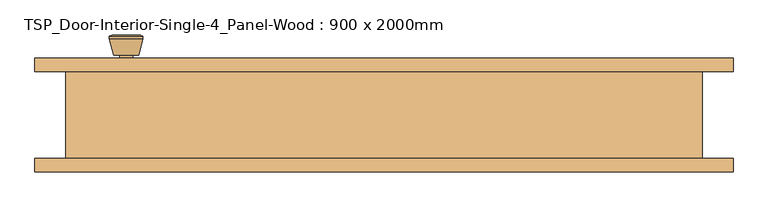
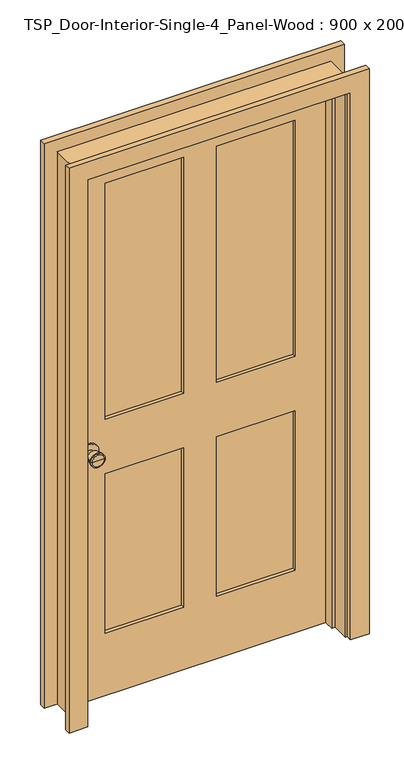
"""IFC4 building model written with IfcOpenShell, lengths in millimetres: door geometry, TSP_Door-Interior-Single-4_Panel-Wood : 900 x 2000mm."""

from ifc_helpers import new_model, si_unit, point, frame, frame_2d, origin, place, context, project, spatial, polyline, circle_curve, trimmed, segment, composite_curve, outline, extrude, faceted_brep, source, transform, mapped, element, save
from ifc_brep_helpers import plane_surface, cylinder_surface, revolved_surface, advanced_brep


def tsp_door_interior_single_4_panel_wood_900_x_2000mm_5c8e3635(model_context):
    return source(origin(), model_context, "Body", "SolidModel", [
        advanced_brep(
        [(-385.0, 20.825, 914.4), (-375.0, 20.825, 914.4), (-395.0, 20.825, 914.4), (-364.5241324, -28.175, 914.4), (-385.0, -28.175, 914.4), (-405.4758676, -28.175, 914.4), (-360.0, -26.3471319, 914.4), (-410.0, -26.3471319, 914.4), (-360.0, -22.8834537, 914.4), (-410.0, -22.8834537, 914.4), (-366.363764, 1.825, 914.4), (-403.636236, 1.825, 914.4), (-375.0, 1.825, 914.4), (-395.0, 1.825, 914.4)],
        [
            (0, 1),
            (1, 2, circle_curve(frame((-385.0, 20.825, 914.4), z_axis=(0.0, 1.0, 0.0), x_axis=(-1.0, 0.0, 0.0)), 10.0)),
            (2, 0),
            (2, 1, circle_curve(frame((-385.0, 20.825, 914.4), z_axis=(0.0, 1.0, 0.0), x_axis=(-1.0, 0.0, 0.0)), 10.0)),
            (3, 4),
            (4, 5),
            (5, 3, circle_curve(frame((-385.0, -28.175, 914.4), z_axis=(0.0, -1.0, 0.0), x_axis=(-1.0, 0.0, 0.0)), 20.4758676)),
            (3, 5, circle_curve(frame((-385.0, -28.175, 914.4), z_axis=(0.0, -1.0, 0.0), x_axis=(-1.0, 0.0, 0.0)), 20.4758676)),
            (6, 3),
            (5, 7),
            (7, 6, circle_curve(frame((-385.0, -26.3471319, 914.4), z_axis=(0.0, -1.0, 0.0), x_axis=(-1.0, 0.0, 0.0)), 25.0)),
            (6, 7, circle_curve(frame((-385.0, -26.3471319, 914.4), z_axis=(0.0, -1.0, 0.0), x_axis=(-1.0, 0.0, 0.0)), 25.0)),
            (8, 6),
            (7, 9),
            (9, 8, circle_curve(frame((-385.0, -22.8834537, 914.4), z_axis=(0.0, -1.0, 0.0), x_axis=(-1.0, 0.0, 0.0)), 25.0)),
            (8, 9, circle_curve(frame((-385.0, -22.8834537, 914.4), z_axis=(0.0, -1.0, 0.0), x_axis=(-1.0, 0.0, 0.0)), 25.0)),
            (10, 8),
            (9, 11),
            (11, 10, circle_curve(frame((-385.0, 1.825, 914.4), z_axis=(0.0, -1.0, 0.0), x_axis=(-1.0, 0.0, 0.0)), 18.636236)),
            (10, 11, circle_curve(frame((-385.0, 1.825, 914.4), z_axis=(0.0, -1.0, 0.0), x_axis=(-1.0, 0.0, 0.0)), 18.636236)),
            (12, 10),
            (11, 13),
            (13, 12, circle_curve(frame((-385.0, 1.825, 914.4), z_axis=(0.0, -1.0, 0.0), x_axis=(-1.0, 0.0, 0.0)), 10.0)),
            (12, 13, circle_curve(frame((-385.0, 1.825, 914.4), z_axis=(0.0, -1.0, 0.0), x_axis=(-1.0, 0.0, 0.0)), 10.0)),
            (1, 12),
            (13, 2),
        ],
        [
            plane_surface(frame((-385.0, 20.825, 914.4), z_axis=(0.0, 1.0, 0.0), x_axis=(-1.0, 0.0, 0.0))),
            plane_surface(frame((-385.0, -28.175, 914.4), z_axis=(0.0, -1.0, 0.0), x_axis=(-1.0, 0.0, 0.0))),
            revolved_surface(polyline([(-405.4758676, -28.175, 914.4), (-410.0, -26.3471319, 914.4)]), (-385.0, 20.825, 914.4), (0.0, 1.0, 0.0)),
            cylinder_surface(frame((-385.0, 20.825, 914.4), z_axis=(0.0, 1.0, 0.0), x_axis=(-1.0, 0.0, 0.0)), 25.0),
            revolved_surface(polyline([(-410.0, -22.8834537, 914.4), (-403.636236, 1.825, 914.4)]), (-385.0, 20.825, 914.4), (0.0, 1.0, 0.0)),
            plane_surface(frame((-385.0, 1.825, 914.4), z_axis=(0.0, 1.0, 0.0), x_axis=(-1.0, 0.0, 0.0))),
            cylinder_surface(frame((-385.0, 20.825, 914.4), z_axis=(0.0, 1.0, 0.0), x_axis=(-1.0, 0.0, 0.0)), 10.0),
        ],
        [
            (0, [[1, 2, 3]]),
            (0, [[-3, 4, -1]]),
            (1, [[5, 6, 7]]),
            (1, [[-6, -5, 8]]),
            (2, [[9, -7, 10, 11]]),
            (2, [[-10, -8, -9, 12]]),
            (3, [[13, -11, 14, 15]]),
            (3, [[-14, -12, -13, 16]]),
            (4, [[17, -15, 18, 19]]),
            (4, [[-18, -16, -17, 20]]),
            (5, [[21, -19, 22, 23]]),
            (5, [[-22, -20, -21, 24]]),
            (6, [[25, -23, 26, -2]]),
            (6, [[-26, -24, -25, -4]]),
        ],
    ),
        extrude(outline(composite_curve([segment(trimmed(circle_curve(frame_2d((914.4, -385.0)), 30.0), [point((914.4, -415.0))], [point((914.4, -355.0))], False, "CARTESIAN"), True, "CONTINUOUS"), segment(trimmed(circle_curve(frame_2d((914.4, -385.0)), 30.0), [point((914.4, -355.0))], [point((914.4, -415.0))], False, "CARTESIAN"), True, "CONTINUOUS")], self_intersect=False)), frame((0.0, 20.825, 0.0), z_axis=(0.0, 1.0, 0.0), x_axis=(0.0, 0.0, 1.0)), (0.0, 0.0, 1.0), 6.0),
        advanced_brep(
        [(-385.0, 67.825, 914.4), (-395.0, 67.825, 914.4), (-375.0, 67.825, 914.4), (-364.5241324, 116.825, 914.4), (-405.4758676, 116.825, 914.4), (-385.0, 116.825, 914.4), (-360.0, 114.9971319, 914.4), (-410.0, 114.9971319, 914.4), (-360.0, 111.5334537, 914.4), (-410.0, 111.5334537, 914.4), (-366.363764, 86.825, 914.4), (-403.636236, 86.825, 914.4), (-375.0, 86.825, 914.4), (-395.0, 86.825, 914.4)],
        [
            (0, 1),
            (1, 2, circle_curve(frame((-385.0, 67.825, 914.4), z_axis=(0.0, -1.0, 0.0), x_axis=(-1.0, 0.0, 0.0)), 10.0)),
            (2, 0),
            (2, 1, circle_curve(frame((-385.0, 67.825, 914.4), z_axis=(0.0, -1.0, 0.0), x_axis=(-1.0, 0.0, 0.0)), 10.0)),
            (3, 4, circle_curve(frame((-385.0, 116.825, 914.4), z_axis=(0.0, 1.0, 0.0), x_axis=(-1.0, 0.0, 0.0)), 20.4758676)),
            (4, 5),
            (5, 3),
            (4, 3, circle_curve(frame((-385.0, 116.825, 914.4), z_axis=(0.0, 1.0, 0.0), x_axis=(-1.0, 0.0, 0.0)), 20.4758676)),
            (6, 7, circle_curve(frame((-385.0, 114.9971319, 914.4), z_axis=(0.0, 1.0, 0.0), x_axis=(-1.0, 0.0, 0.0)), 25.0)),
            (7, 4),
            (3, 6),
            (7, 6, circle_curve(frame((-385.0, 114.9971319, 914.4), z_axis=(0.0, 1.0, 0.0), x_axis=(-1.0, 0.0, 0.0)), 25.0)),
            (8, 9, circle_curve(frame((-385.0, 111.5334537, 914.4), z_axis=(0.0, 1.0, 0.0), x_axis=(-1.0, 0.0, 0.0)), 25.0)),
            (9, 7),
            (6, 8),
            (9, 8, circle_curve(frame((-385.0, 111.5334537, 914.4), z_axis=(0.0, 1.0, 0.0), x_axis=(-1.0, 0.0, 0.0)), 25.0)),
            (10, 11, circle_curve(frame((-385.0, 86.825, 914.4), z_axis=(0.0, 1.0, 0.0), x_axis=(-1.0, 0.0, 0.0)), 18.636236)),
            (11, 9),
            (8, 10),
            (11, 10, circle_curve(frame((-385.0, 86.825, 914.4), z_axis=(0.0, 1.0, 0.0), x_axis=(-1.0, 0.0, 0.0)), 18.636236)),
            (12, 13, circle_curve(frame((-385.0, 86.825, 914.4), z_axis=(0.0, 1.0, 0.0), x_axis=(-1.0, 0.0, 0.0)), 10.0)),
            (13, 11),
            (10, 12),
            (13, 12, circle_curve(frame((-385.0, 86.825, 914.4), z_axis=(0.0, 1.0, 0.0), x_axis=(-1.0, 0.0, 0.0)), 10.0)),
            (1, 13),
            (12, 2),
        ],
        [
            plane_surface(frame((-385.0, 67.825, 914.4), z_axis=(0.0, -1.0, 0.0), x_axis=(-1.0, 0.0, 0.0))),
            plane_surface(frame((-385.0, 116.825, 914.4), z_axis=(0.0, 1.0, 0.0), x_axis=(-1.0, 0.0, 0.0))),
            revolved_surface(polyline([(-405.4758676, 116.825, 914.4), (-410.0, 114.9971319, 914.4)]), (-385.0, 67.825, 914.4), (0.0, -1.0, 0.0)),
            cylinder_surface(frame((-385.0, 67.825, 914.4), z_axis=(0.0, -1.0, 0.0), x_axis=(-1.0, 0.0, 0.0)), 25.0),
            revolved_surface(polyline([(-410.0, 111.5334537, 914.4), (-403.636236, 86.825, 914.4)]), (-385.0, 67.825, 914.4), (0.0, -1.0, 0.0)),
            plane_surface(frame((-385.0, 86.825, 914.4), z_axis=(0.0, -1.0, 0.0), x_axis=(-1.0, 0.0, 0.0))),
            cylinder_surface(frame((-385.0, 67.825, 914.4), z_axis=(0.0, -1.0, 0.0), x_axis=(-1.0, 0.0, 0.0)), 10.0),
        ],
        [
            (0, [[1, 2, 3]]),
            (0, [[-3, 4, -1]]),
            (1, [[5, 6, 7]]),
            (1, [[8, -7, -6]]),
            (2, [[9, 10, -5, 11]]),
            (2, [[12, -11, -8, -10]]),
            (3, [[13, 14, -9, 15]]),
            (3, [[16, -15, -12, -14]]),
            (4, [[17, 18, -13, 19]]),
            (4, [[20, -19, -16, -18]]),
            (5, [[21, 22, -17, 23]]),
            (5, [[24, -23, -20, -22]]),
            (6, [[-2, 25, -21, 26]]),
            (6, [[-4, -26, -24, -25]]),
        ],
    ),
        extrude(outline(composite_curve([segment(trimmed(circle_curve(frame_2d((914.4, -385.0)), 30.0), [point((914.4, -415.0))], [point((914.4, -355.0))], False, "CARTESIAN"), True, "CONTINUOUS"), segment(trimmed(circle_curve(frame_2d((914.4, -385.0)), 30.0), [point((914.4, -355.0))], [point((914.4, -415.0))], False, "CARTESIAN"), True, "CONTINUOUS")], self_intersect=False)), frame((0.0, 61.825, 0.0), z_axis=(0.0, 1.0, 0.0), x_axis=(0.0, 0.0, 1.0)), (0.0, 0.0, 1.0), 6.0),
        faceted_brep([(475.0, 61.825, 0.0), (475.0, -68.175, 0.0), (450.0, -68.175, 0.0), (450.0, -8.1, 0.0), (437.3, -8.1, 0.0), (437.3, 26.825, 0.0), (450.0, 26.825, 0.0), (450.0, 61.825, 0.0), (475.0, 61.825, 2025.0), (475.0, -68.175, 2025.0), (-475.0, -68.175, 2025.0), (-475.0, -68.175, 0.0), (-450.0, -68.175, 0.0), (-450.0, -68.175, 2000.0), (450.0, -68.175, 2000.0), (450.0, -8.1, 2000.0), (-450.0, -8.1, 2000.0), (-450.0, -8.1, 0.0), (-437.3, -8.1, 0.0), (-437.3, -8.1, 1987.3), (437.3, -8.1, 1987.3), (437.3, 26.825, 1987.3), (-437.3, 26.825, 1987.3), (-437.3, 26.825, 0.0), (-450.0, 26.825, 0.0), (-450.0, 26.825, 2000.0), (450.0, 26.825, 2000.0), (450.0, 61.825, 2000.0), (-450.0, 61.825, 2000.0), (-450.0, 61.825, 0.0), (-475.0, 61.825, 0.0), (-475.0, 61.825, 2025.0)], [[[0, 1, 2, 3, 4, 5, 6, 7]], [[1, 0, 8, 9]], [[2, 1, 9, 10, 11, 12, 13, 14]], [[3, 2, 14, 15]], [[4, 3, 15, 16, 17, 18, 19, 20]], [[5, 4, 20, 21]], [[6, 5, 21, 22, 23, 24, 25, 26]], [[7, 6, 26, 27]], [[0, 7, 27, 28, 29, 30, 31, 8]], [[9, 8, 31, 10]], [[15, 14, 13, 16]], [[21, 20, 19, 22]], [[27, 26, 25, 28]], [[30, 29, 24, 23, 18, 17, 12, 11]], [[10, 31, 30, 11]], [[16, 13, 12, 17]], [[22, 19, 18, 23]], [[28, 25, 24, 29]]]),
        extrude(outline(polyline([(2000.0, -450.0), (0.0, -450.0), (0.0, 450.0), (2000.0, 450.0), (2000.0, -450.0)]), holes=[polyline([(1880.0, 57.5), (1880.0, 330.0), (1014.4, 330.0), (1014.4, 57.5), (1880.0, 57.5)]), polyline([(1014.4, -57.5), (1014.4, -330.0), (1880.0, -330.0), (1880.0, -57.5), (1014.4, -57.5)]), polyline([(814.4, 57.5), (814.4, 330.0), (230.0, 330.0), (230.0, 57.5), (814.4, 57.5)]), polyline([(230.0, -57.5), (230.0, -330.0), (814.4, -330.0), (814.4, -57.5), (230.0, -57.5)])]), frame((0.0, 26.825, 0.0), z_axis=(0.0, 1.0, 0.0), x_axis=(0.0, 0.0, 1.0)), (0.0, 0.0, 1.0), 35.0),
        extrude(outline(polyline([(330.0, 38.4916667), (57.5, 38.4916667), (57.5, 50.1583333), (330.0, 50.1583333), (330.0, 38.4916667)])), frame((0.0, 0.0, 1014.4), z_axis=(0.0, 0.0, 1.0), x_axis=(1.0, 0.0, 0.0)), (0.0, 0.0, 1.0), 865.6),
        extrude(outline(polyline([(-57.5, 38.4916667), (-330.0, 38.4916667), (-330.0, 50.1583333), (-57.5, 50.1583333), (-57.5, 38.4916667)])), frame((0.0, 0.0, 1014.4), z_axis=(0.0, 0.0, 1.0), x_axis=(1.0, 0.0, 0.0)), (0.0, 0.0, 1.0), 865.6),
        extrude(outline(polyline([(330.0, 38.4916667), (57.5, 38.4916667), (57.5, 50.1583333), (330.0, 50.1583333), (330.0, 38.4916667)])), frame((0.0, 0.0, 230.0), z_axis=(0.0, 0.0, 1.0), x_axis=(1.0, 0.0, 0.0)), (0.0, 0.0, 1.0), 584.4),
        extrude(outline(polyline([(-57.5, 38.4916667), (-330.0, 38.4916667), (-330.0, 50.1583333), (-57.5, 50.1583333), (-57.5, 38.4916667)])), frame((0.0, 0.0, 230.0), z_axis=(0.0, 0.0, 1.0), x_axis=(1.0, 0.0, 0.0)), (0.0, 0.0, 1.0), 584.4),
        extrude(outline(polyline([(0.0, 456.35), (0.0, 521.35), (2071.35, 521.35), (2071.35, -521.35), (0.0, -521.35), (0.0, -456.35), (2006.35, -456.35), (2006.35, 456.35), (0.0, 456.35)])), frame((0.0, 61.825, 0.0), z_axis=(0.0, 1.0, 0.0), x_axis=(0.0, 0.0, 1.0)), (0.0, 0.0, 1.0), 20.0),
        extrude(outline(polyline([(0.0, 456.35), (0.0, 521.35), (2071.35, 521.35), (2071.35, -521.35), (0.0, -521.35), (0.0, -456.35), (2006.35, -456.35), (2006.35, 456.35), (0.0, 456.35)])), frame((0.0, -88.175, 0.0), z_axis=(0.0, 1.0, 0.0), x_axis=(0.0, 0.0, 1.0)), (0.0, 0.0, 1.0), 20.0),
    ])


if __name__ == "__main__":
    model = new_model("IFC4")
    model_context = context("Model", 3, world=origin())
    ifc_project = project(units=[si_unit("LENGTHUNIT", "METRE", prefix="MILLI")], contexts=[model_context])
    site = spatial("IfcSite", under=ifc_project)
    building = spatial("IfcBuilding", under=site)
    placement = place(None, origin())
    tsp_door_interior_single_4_panel_wood_900_x_2000mm_shape = tsp_door_interior_single_4_panel_wood_900_x_2000mm_5c8e3635(model_context)
    element("IfcDoor", 1, ObjectType="TSP_Door-Interior-Single-4_Panel-Wood : 900 x 2000mm", at=placement, inside=building, context=model_context, shape_type="MappedRepresentation", body=[
        mapped(tsp_door_interior_single_4_panel_wood_900_x_2000mm_shape, transform((0.0, 0.0, 0.0), x_axis=(1.0, 0.0, 0.0), y_axis=(0.0, 1.0, 0.0), z_axis=(0.0, 0.0, 1.0))),
    ])
    save(model, "model.ifc")

# Revit data of these elements
# Type "TSP_Door-Interior-Single-4_Panel-Wood : 900 x 2000mm"
#   Model = "TSP_DOOR02W"
#   Type Mark = "231"
#   Assembly Code = "C1020300"
#   Analytic Construction = "Wooden"
#   Top Rail = 120 mm
#   Thickness = 35 mm
#   Thermal Resistance (R) = 0.455703 (m²·K)/W
#   Swing Angle [instance default] = 90.00°
#   Stiles = 120 mm
#   Rough Width = 950 mm
#   Rough Height = 2025 mm
#   Mullion = 115 mm
#   Lock Rail = 200 mm
#   Height = 2000 mm
#   Width = 900 mm
#   Heat Transfer Coefficient (U) = 2.19465 W/(m²·K)
#   Bottom Rail = 230 mm
#   Define Thermal Properties by = 1
#   Trim Material = Cherry
#   Panel Material = Cherry
#   Frame Material = Cherry
#   Door Handle Material = Aluminum
#   Visual Light Transmittance = 0
#   Solar Heat Gain Coefficient = 0
#   Wall Closure = (empty or 0)
#   Function = (empty or 0)
# Element 1 (IfcDoor, "TSP_Door-Interior-Single-4_Panel-Wood : 900 x 2000mm")
#   Materials on its faces: "Cherry", "Aluminum"
# Materials
#   "Cherry": class "Wood", colour RGB 226 177 128, transparency 0, Description = "Prunus Serotina", Cost = 0
#   "Aluminum": class "Metal", colour RGB 247 247 247, transparency 0, Description = "Aluminum 6061", Cost = 0
